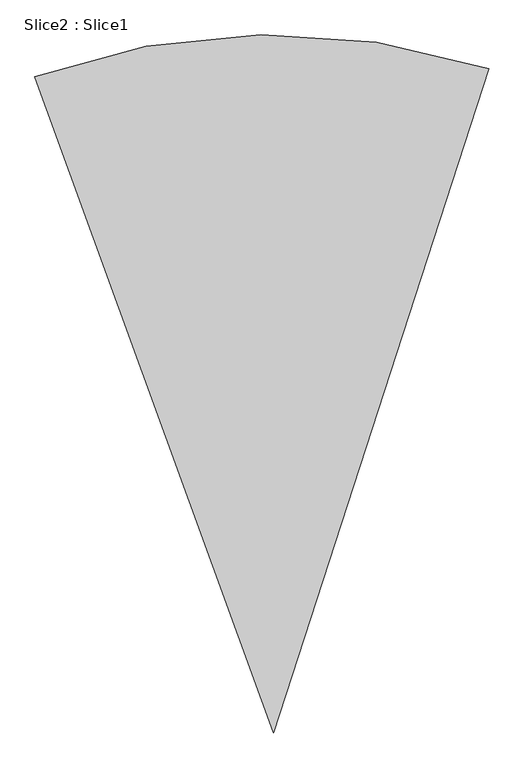
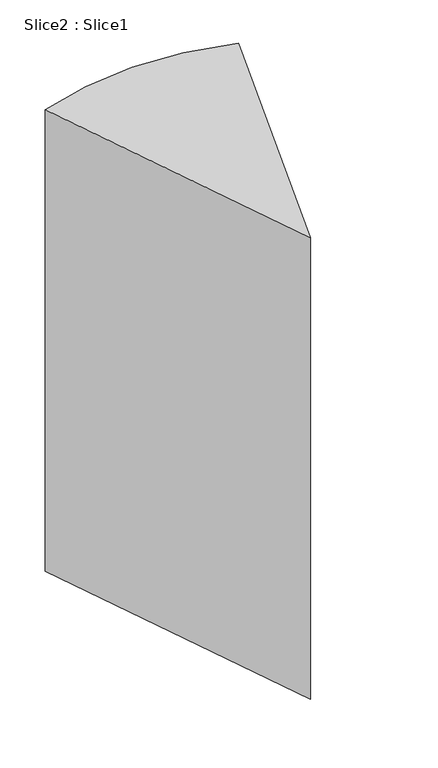
"""IFC4 building model written with IfcOpenShell, lengths in millimetres: proxy geometry, Slice2 : Slice1."""

from ifc_helpers import new_model, si_unit, point, origin, origin_with_axes, origin_2d, place, context, project, spatial, polyline, circle_curve, trimmed, segment, composite_curve, outline, extrude, source, transform, mapped, element, save


def slice2_slice1_1b8b2f56(model_context):
    return source(origin(), model_context, "Body", "SweptSolid", [
        extrude(outline(composite_curve([segment(polyline([(339.9186938, 1046.1621679), (0.0, 0.0), (-376.2221577, 1033.6618829)]), True, "CONTINUOUS"), segment(trimmed(circle_curve(origin_2d(), 1100.0), [point((-376.2221577, 1033.6618829))], [point((339.9186938, 1046.1621679))], False, "CARTESIAN"), True, "CONTINUOUS")], self_intersect=False)), origin_with_axes(), (0.0, 0.0, 1.0), 1790.564951),
    ])


if __name__ == "__main__":
    model = new_model("IFC4")
    model_context = context("Model", 3, world=origin())
    ifc_project = project(units=[si_unit("LENGTHUNIT", "METRE", prefix="MILLI")], contexts=[model_context])
    site = spatial("IfcSite", under=ifc_project)
    building = spatial("IfcBuilding", under=site)
    placement = place(None, origin())
    slice2_slice1_shape = slice2_slice1_1b8b2f56(model_context)
    element("IfcBuildingElementProxy", 1, Name="Slice2 : Slice1", ObjectType="Slice2 : Slice1", at=placement, inside=building, context=model_context, shape_type="MappedRepresentation", body=[
        mapped(slice2_slice1_shape, transform((0.0, 0.0, 0.0), x_axis=(1.0, 0.0, 0.0), y_axis=(0.0, 1.0, 0.0), z_axis=(0.0, 0.0, 1.0))),
    ])
    save(model, "model.ifc")

# Revit data of these elements
# Project information
#   Organization Name = "EWP"
#   Author = "Tecx"
#   EWP_Sheet_Originator Code = "EWP"
#   EWP_Sheet_Role Code = "S"
#   EWP_Project_BIM Contact = "BIMx"
#   EWP_Project_BIM Number = "BIMBIM"
#   EWP_Project_Revit Version = "2022"
#   EWP_Project_Service Engineer = "j"
#   EWP_Project_Surveyor = "h"
#   Project Status = "Preliminary"
#   Client Name = "Client"
#   Project Address = "35 This Project Stays in The Office"
#   Project Name = "A New Template"
#   Project Number = "2022123"
